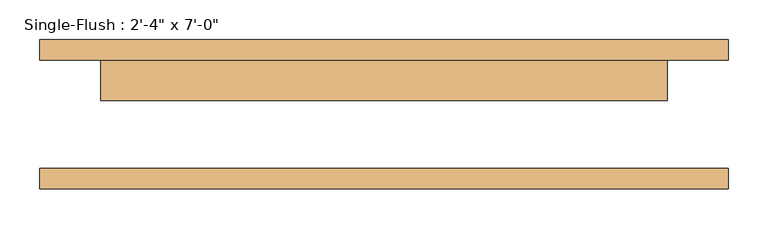
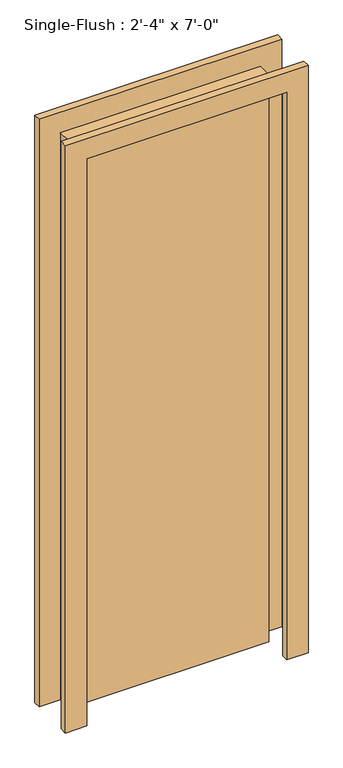
"""IFC4 building model written with IfcOpenShell, lengths in millimetres: door geometry."""

from ifc_helpers import new_model, si_unit, frame, origin, origin_with_axes, place, context, project, spatial, polyline, outline, extrude, source, transform, mapped, element, save


def door_eeaf238e(model_context):
    return source(origin(), model_context, "Body", "SweptSolid", [
        extrude(outline(polyline([(2209.8, -431.8), (0.0, -431.8), (0.0, -355.6), (2133.6, -355.6), (2133.6, 355.6), (0.0, 355.6), (0.0, 431.8), (2209.8, 431.8), (2209.8, -431.8)])), frame((0.0, 68.2625, 0.0), z_axis=(0.0, 1.0, 0.0), x_axis=(0.0, 0.0, 1.0)), (0.0, 0.0, 1.0), 25.4),
        extrude(outline(polyline([(2209.8, 431.8), (2209.8, -431.8), (0.0, -431.8), (0.0, -355.6), (2133.6, -355.6), (2133.6, 355.6), (0.0, 355.6), (0.0, 431.8), (2209.8, 431.8)])), frame((0.0, -93.6625, 0.0), z_axis=(0.0, 1.0, 0.0), x_axis=(0.0, 0.0, 1.0)), (0.0, 0.0, 1.0), 25.4),
        extrude(outline(polyline([(355.6, 17.4625), (-355.6, 17.4625), (-355.6, 68.2625), (355.6, 68.2625), (355.6, 17.4625)])), origin_with_axes(), (0.0, 0.0, 1.0), 2133.6),
    ])


if __name__ == "__main__":
    model = new_model("IFC4")
    model_context = context("Model", 3, world=origin())
    ifc_project = project(units=[si_unit("LENGTHUNIT", "METRE", prefix="MILLI")], contexts=[model_context])
    site = spatial("IfcSite", under=ifc_project)
    building = spatial("IfcBuilding", under=site)
    placement = place(None, origin())
    door_shape = door_eeaf238e(model_context)
    element("IfcDoor", 1, ObjectType="Single-Flush : 2'-4\" x 7'-0\"", at=placement, inside=building, context=model_context, shape_type="MappedRepresentation", body=[
        mapped(door_shape, transform((0.0, 0.0, 0.0), x_axis=(1.0, 0.0, 0.0), y_axis=(0.0, 1.0, 0.0), z_axis=(0.0, 0.0, 1.0))),
    ])
    save(model, "model.ifc")

# Revit data of these elements
# Type "Single-Flush : 2'-4\" x 7'-0\""
#   Type Mark = "8"
#   Construction Type Id = "MDOOR"
#   Assembly Code = "C1020"
#   Analytic Construction = "Metal"
#   Thickness = 0' - 2"
#   Heat Transfer Coefficient (U) = 3.7021 W/(m²·K)
#   Height = 7' - 0"
#   Trim Projection Ext = 0' - 1"
#   Trim Projection Int = 0' - 1"
#   Trim Width = 0' - 3"
#   Width = 2' - 4"
#   Door Material = Door - Panel
#   Frame Material = Door - Frame
#   Visual Light Transmittance = 0
#   Solar Heat Gain Coefficient = 0
#   Function = (empty or 0)
#   Wall Closure = (empty or 0)
# Element 1 (IfcDoor, "Single-Flush : 2'-4\" x 7'-0\"")
#   Materials on its faces: "Door - Frame", "Door - Panel"
# Materials
#   "Door - Panel": class "Wood", colour RGB 210 159 95, transparency 0, Cost = 0
#   "Door - Frame": class "Miscellaneous", colour RGB 118 70 51, transparency 0, Cost = 0
